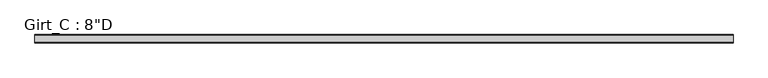
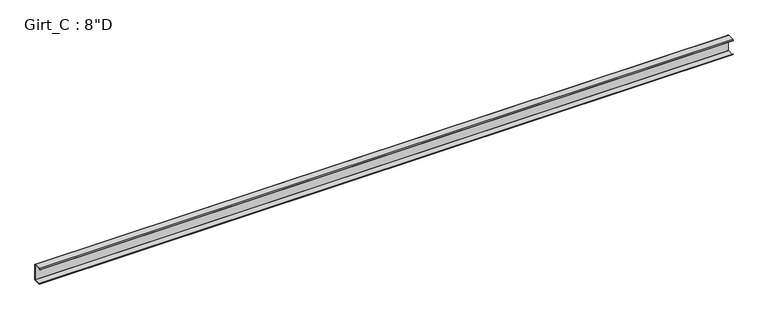
"""IFC4 building model written with IfcOpenShell, lengths in millimetres: beam geometry."""

import ifcopenshell
import ifcopenshell.guid

model = None  # the IFC model being written
_history = None  # IfcOwnerHistory: only IFC2X3 demands one
_inside = {}  # id of a spatial element -> (the spatial element, [elements in it])
_under = {}  # id of a project, library or spatial element -> (it, [spatial elements below it])
_declared = {}  # id of a project -> (the project, [libraries it declares])
_typed = {}  # id of a type object -> (the type object, [elements of that type])
_made_of = {}  # id of a material, layer set ... -> (it, [elements and type objects made of it])


def new_model(schema):
    """Start an empty IFC model of exactly this schema.

    Asked for "IFC4X3", IfcOpenShell would pick the latest addendum, in which some entities
    have other attributes; the version numbers below select the first issue.
    IFC2X3 requires an IfcOwnerHistory on every rooted entity: one is made here for all.
    """
    global model, _history
    if schema == "IFC4X3":
        model = ifcopenshell.file(schema_version=(4, 3, 0, 0))
    else:
        model = ifcopenshell.file(schema=schema)
    _inside.clear()
    _under.clear()
    _declared.clear()
    _typed.clear()
    _made_of.clear()
    _history = None
    if model.schema == "IFC2X3":
        org = make("IfcOrganization", Name="unknown")
        user = make(
            "IfcPersonAndOrganization",
            ThePerson=make("IfcPerson", FamilyName="unknown"),
            TheOrganization=org,
        )
        app = make(
            "IfcApplication",
            ApplicationDeveloper=org,
            Version="unknown",
            ApplicationFullName="unknown",
            ApplicationIdentifier="unknown",
        )
        _history = make(
            "IfcOwnerHistory",
            OwningUser=user,
            OwningApplication=app,
            ChangeAction="ADDED",
            CreationDate=0,
        )
    return model


def make(cls, **values):
    """One entity of the class cls with the attributes given. An attribute that is None is left unset."""
    return model.create_entity(
        cls, **{name: value for name, value in values.items() if value is not None}
    )


def rooted(cls, **values):
    """An entity with a GlobalId (a new one), such as an element, a storey or a relation."""
    return make(cls, GlobalId=ifcopenshell.guid.new(), OwnerHistory=_history, **values)


def si_unit(unit_type, name, prefix=None):
    """IfcSIUnit, for example si_unit("LENGTHUNIT", "METRE", prefix="MILLI")."""
    return make("IfcSIUnit", UnitType=unit_type, Prefix=prefix, Name=name)


def assignment(units):
    """IfcUnitAssignment: the units of a project."""
    return None if units is None else make("IfcUnitAssignment", Units=units)


def point(xyz):
    """IfcCartesianPoint."""
    return None if xyz is None else make("IfcCartesianPoint", Coordinates=xyz)


def direction(xyz):
    """IfcDirection."""
    return None if xyz is None else make("IfcDirection", DirectionRatios=xyz)


def frame(location, z_axis=None, x_axis=None):
    """IfcAxis2Placement3D, a coordinate frame: its origin and axes. An axis left out is left unset."""
    return make(
        "IfcAxis2Placement3D",
        Location=point(location),
        Axis=direction(z_axis),
        RefDirection=direction(x_axis),
    )


def frame_2d(location, x_axis=None):
    """IfcAxis2Placement2D, a coordinate frame in the plane: its origin and x axis."""
    return make(
        "IfcAxis2Placement2D", Location=point(location), RefDirection=direction(x_axis)
    )


def origin():
    """The frame at (0, 0, 0) with its axes left unset."""
    return frame((0.0, 0.0, 0.0))


def place(relative_to, where):
    """IfcLocalPlacement: puts the frame where relative to a parent placement (None: the world)."""
    return make(
        "IfcLocalPlacement", PlacementRelTo=relative_to, RelativePlacement=where
    )


def context(
    kind, dimensions, precision=None, world=None, true_north=None, identifier=None
):
    """IfcGeometricRepresentationContext, for example the 3D "Model" context."""
    return make(
        "IfcGeometricRepresentationContext",
        ContextIdentifier=identifier,
        ContextType=kind,
        CoordinateSpaceDimension=dimensions,
        Precision=precision,
        WorldCoordinateSystem=world,
        TrueNorth=true_north,
    )


def project(units=None, contexts=None):
    """IfcProject with its units and contexts."""
    return rooted(
        "IfcProject",
        Name="project",
        RepresentationContexts=contexts,
        UnitsInContext=assignment(units),
    )


def spatial(cls, under=None, at=None, **own):
    """A site, building, storey or space (cls), placed at a placement, below another one or the project."""
    s = rooted(cls, ObjectPlacement=at, **own)
    if under is not None:
        _under.setdefault(under.id(), (under, []))[1].append(s)
    return s


def polyline(points):
    """IfcPolyline through the points."""
    return make("IfcPolyline", Points=[point(p) for p in points])


def circle_curve(where, radius):
    """IfcCircle in the frame where."""
    return make("IfcCircle", Position=where, Radius=radius)


def trimmed(basis, trim1, trim2, sense, master):
    """IfcTrimmedCurve: the piece of a basis curve between two trims."""
    return make(
        "IfcTrimmedCurve",
        BasisCurve=basis,
        Trim1=trim1,
        Trim2=trim2,
        SenseAgreement=sense,
        MasterRepresentation=master,
    )


def segment(curve, same_sense, transition):
    """IfcCompositeCurveSegment."""
    return make(
        "IfcCompositeCurveSegment",
        Transition=transition,
        SameSense=same_sense,
        ParentCurve=curve,
    )


def composite_curve(segments, self_intersect=None):
    """IfcCompositeCurve: segments joined end to end."""
    return make("IfcCompositeCurve", Segments=segments, SelfIntersect=self_intersect)


def outline(outer, holes=None, kind="AREA"):
    """IfcArbitraryClosedProfileDef: a profile drawn as a closed curve; with holes, ...WithVoids."""
    if holes is None:
        return make("IfcArbitraryClosedProfileDef", ProfileType=kind, OuterCurve=outer)
    return make(
        "IfcArbitraryProfileDefWithVoids",
        ProfileType=kind,
        OuterCurve=outer,
        InnerCurves=holes,
    )


def extrude(swept, where, along, depth):
    """IfcExtrudedAreaSolid: the profile swept, set in the frame where, extruded along a direction by depth."""
    return make(
        "IfcExtrudedAreaSolid",
        SweptArea=swept,
        Position=where,
        ExtrudedDirection=direction(along),
        Depth=depth,
    )


def shape(context_of_items, identifier, shape_type, items):
    """IfcShapeRepresentation: the items that make up one representation, for example the "Body"."""
    return make(
        "IfcShapeRepresentation",
        ContextOfItems=context_of_items,
        RepresentationIdentifier=identifier,
        RepresentationType=shape_type,
        Items=items,
    )


def source(mapping_origin, context_of_items, identifier, shape_type, items):
    """IfcRepresentationMap: a shape defined once, which mapped items show again and again."""
    return make(
        "IfcRepresentationMap",
        MappingOrigin=mapping_origin,
        MappedRepresentation=shape(context_of_items, identifier, shape_type, items),
    )


def transform(
    local_origin,
    x_axis=None,
    y_axis=None,
    z_axis=None,
    scale=None,
    scale2=None,
    scale3=None,
    uniform=True,
):
    """IfcCartesianTransformationOperator3D, or its non-uniform kind. x_axis, y_axis, z_axis: its Axis1, 2, 3."""
    if uniform:
        return make(
            "IfcCartesianTransformationOperator3D",
            Axis1=direction(x_axis),
            Axis2=direction(y_axis),
            LocalOrigin=point(local_origin),
            Scale=scale,
            Axis3=direction(z_axis),
        )
    return make(
        "IfcCartesianTransformationOperator3DnonUniform",
        Axis1=direction(x_axis),
        Axis2=direction(y_axis),
        LocalOrigin=point(local_origin),
        Scale=scale,
        Axis3=direction(z_axis),
        Scale2=scale2,
        Scale3=scale3,
    )


def mapped(mapping_source, mapping_target):
    """IfcMappedItem: shows the shape of a source again, moved by a transform."""
    return make(
        "IfcMappedItem", MappingSource=mapping_source, MappingTarget=mapping_target
    )


def made_of(thing, what):
    """Note that an element or type object is made of a material, layer set ...; save() writes the relation."""
    if what is not None:
        _made_of.setdefault(what.id(), (what, []))[1].append(thing)
    return thing


def element(
    cls,
    number,
    at=None,
    inside=None,
    cuts=None,
    type_object=None,
    material=None,
    context=None,
    identifier="Body",
    shape_type=None,
    held_by="IfcProductDefinitionShape",
    body=None,
    shapes=None,
    **own,
):
    """One element of the class cls, such as IfcWall. Its Tag is "e" and its number.

    at: its placement. inside: the storey or other place that contains it. cuts: it is an
    opening in that element (IfcRelVoidsElement). A single representation is given by context,
    identifier, shape_type and body (its items); several are given by shapes. held_by: the class
    of the entity that holds the representations. save() writes the other relations.
    """
    e = rooted(cls, Tag="e%d" % number, ObjectPlacement=at, **own)
    if body is not None:
        shapes = [shape(context, identifier, shape_type, body)]
    if shapes is not None:
        e.Representation = make(held_by, Representations=shapes)
    if inside is not None:
        _inside.setdefault(inside.id(), (inside, []))[1].append(e)
    if cuts is not None:
        rooted(
            "IfcRelVoidsElement", RelatingBuildingElement=cuts, RelatedOpeningElement=e
        )
    if type_object is not None:
        _typed.setdefault(type_object.id(), (type_object, []))[1].append(e)
    return made_of(e, material)


def aggregate(whole, parts):
    """IfcRelAggregates: a whole, such as a stair, and the parts it consists of."""
    return rooted("IfcRelAggregates", RelatingObject=whole, RelatedObjects=parts)


def save(model, path):
    """Write the relations noted so far, then the file.

    IfcRelAggregates (storeys below a building ...), IfcRelContainedInSpatialStructure (elements
    in a storey), IfcRelDefinesByType, IfcRelAssociatesMaterial and IfcRelDeclares: one each for
    every whole, place, type object, material and project.
    """
    for whole, parts in _under.values():
        aggregate(whole, parts)
    for where, things in _inside.values():
        rooted(
            "IfcRelContainedInSpatialStructure",
            RelatedElements=things,
            RelatingStructure=where,
        )
    for kind, things in _typed.values():
        rooted("IfcRelDefinesByType", RelatedObjects=things, RelatingType=kind)
    for what, things in _made_of.values():
        rooted("IfcRelAssociatesMaterial", RelatedObjects=things, RelatingMaterial=what)
    for by, libraries in _declared.values():
        rooted("IfcRelDeclares", RelatingContext=by, RelatedDefinitions=libraries)
    model.write(path)


def beam_f332ffda(model_context):
    return source(origin(), model_context, "Body", "SweptSolid", [
        extrude(outline(composite_curve([segment(polyline([(-87.5109375, 101.6), (-3.3734375, 101.6)]), True, "CONTINUOUS"), segment(trimmed(circle_curve(frame_2d((-3.3734375, 96.8375)), 4.7625), [point((-3.3734375, 101.6))], [point((1.3890625, 96.8375))], False, "CARTESIAN"), True, "CONTINUOUS"), segment(polyline([(1.3890625, 96.8375), (1.3890625, -96.8375)]), True, "CONTINUOUS"), segment(trimmed(circle_curve(frame_2d((-3.3734375, -96.8375)), 4.7625), [point((1.3890625, -96.8375))], [point((-3.3734375, -101.6))], False, "CARTESIAN"), True, "CONTINUOUS"), segment(polyline([(-3.3734375, -101.6), (-87.5109375, -101.6), (-99.7792647, -86.979177), (-97.6510975, -85.1934327), (-86.2154765, -98.821875), (-3.2694106, -98.821875)]), True, "CONTINUOUS"), segment(trimmed(circle_curve(frame_2d((-3.3748024, -96.8389339)), 1.9857399), [point((-3.2694106, -98.821875))], [point((-1.3890625, -96.8389339))], True, "CARTESIAN"), True, "CONTINUOUS"), segment(polyline([(-1.3890625, -96.8389339), (-1.3890625, 96.8381931)]), True, "CONTINUOUS"), segment(trimmed(circle_curve(frame_2d((-3.3741066, 96.8381931)), 1.9850441), [point((-1.3890625, 96.8381931))], [point((-3.3005807, 98.821875))], True, "CARTESIAN"), True, "CONTINUOUS"), segment(polyline([(-3.3005807, 98.821875), (-86.2154765, 98.821875), (-97.6278742, 85.221109), (-99.7560415, 87.0068534), (-87.5109375, 101.6)]), True, "CONTINUOUS")], self_intersect=False)), frame((-4209.247087, 0.0, 0.0), z_axis=(1.0, 0.0, 0.0), x_axis=(0.0, 1.0, 0.0)), (0.0, 0.0, 1.0), 8416.0185616),
    ])


if __name__ == "__main__":
    model = new_model("IFC4")
    model_context = context("Model", 3, world=origin())
    ifc_project = project(units=[si_unit("LENGTHUNIT", "METRE", prefix="MILLI")], contexts=[model_context])
    site = spatial("IfcSite", under=ifc_project)
    building = spatial("IfcBuilding", under=site)
    placement = place(None, origin())
    beam_shape = beam_f332ffda(model_context)
    element("IfcBeam", 1, ObjectType="Girt_C : 8\"D", at=placement, inside=building, context=model_context, shape_type="MappedRepresentation", body=[
        mapped(beam_shape, transform((0.0, 0.0, 0.0), x_axis=(1.0, 0.0, 0.0), y_axis=(0.0, 1.0, 0.0), z_axis=(0.0, 0.0, 1.0))),
    ])
    save(model, "model.ifc")

# Revit data of these elements
# Type "Girt_C : 8\"D"
#   half leg = 0' - 1 3/4"
#   Web_Thickness = 0' - 0 7/64"
#   Length [instance default] = 10' - 0"
#   Leg_1 = 0' - 3 1/2"
#   Height = 0' - 8"
#   Structural Material [instance default] = none
# Element 1 (IfcBeam, "Girt_C : 8\"D")
#   Structural Material = CEE' SECTION (8.0x3.5C - SEE STRUCT. DWGS)
#   Materials on its faces: "CEE' SECTION (8.0x3.5C - SEE STRUCT. DWGS)"
# Materials
#   "CEE' SECTION (8.0x3.5C - SEE STRUCT. DWGS)": class "Metal", colour RGB 137 146 153, transparency 0, Description = "Steel, mill finish", Cost = 0
